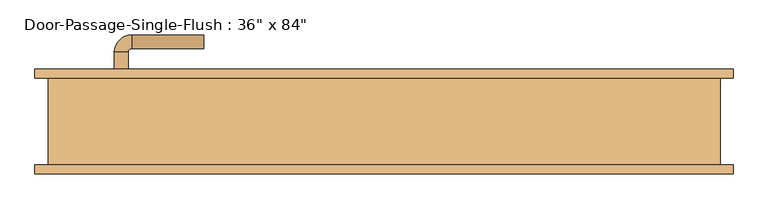
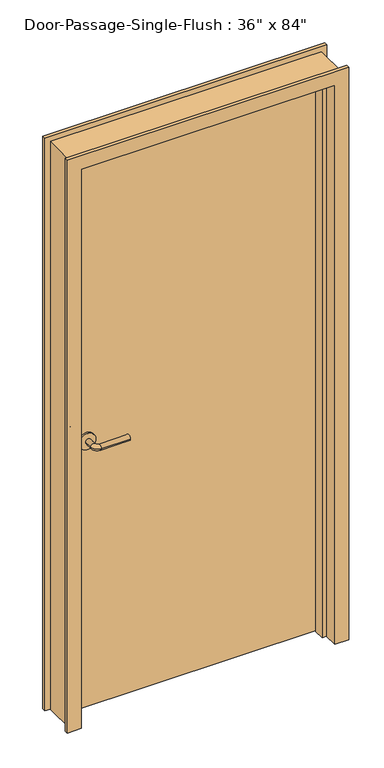
"""IFC4 building model written with IfcOpenShell, lengths in millimetres: door geometry."""

from ifc_helpers import new_model, si_unit, point, frame, frame_2d, origin, origin_with_axes, place, context, project, spatial, polyline, circle_curve, ellipse_curve, trimmed, segment, composite_curve, outline, extrude, faceted_brep, source, transform, mapped, element, save
from ifc_brep_helpers import plane_surface, cylinder_surface, revolved_surface, advanced_brep


def door_12b10c6a(model_context):
    return source(origin(), model_context, "Body", "SolidModel", [
        advanced_brep(
        [(-392.190625, 17.4, 1016.0), (-372.190625, 17.4, 1016.0), (-372.190625, -12.6, 1016.0), (-392.190625, -12.6, 1016.0), (-367.190625, -17.6, 1016.0), (-367.190625, -37.6, 1016.0), (-262.190625, -37.6, 1016.0), (-262.190625, -17.6, 1016.0)],
        [
            (0, 1, circle_curve(frame((-382.190625, 17.4, 1016.0), z_axis=(0.0, 1.0, 0.0), x_axis=(1.0, 0.0, 0.0)), 10.0)),
            (1, 0, circle_curve(frame((-382.190625, 17.4, 1016.0), z_axis=(0.0, 1.0, 0.0), x_axis=(1.0, 0.0, 0.0)), 10.0)),
            (1, 2),
            (2, 3, circle_curve(frame((-382.190625, -12.6, 1016.0), z_axis=(0.0, 1.0, 0.0), x_axis=(1.0, 0.0, 0.0)), 10.0)),
            (3, 0),
            (3, 2, circle_curve(frame((-382.190625, -12.6, 1016.0), z_axis=(0.0, 1.0, 0.0), x_axis=(1.0, 0.0, 0.0)), 10.0)),
            (4, 5, circle_curve(frame((-367.190625, -27.6, 1016.0), z_axis=(-1.0, 0.0, 0.0), x_axis=(0.0, 1.0, 0.0)), 10.0)),
            (5, 3, circle_curve(frame((-367.190625, -12.6, 1016.0), z_axis=(0.0, 0.0, -1.0), x_axis=(-1.0, 0.0, 0.0)), 25.0)),
            (2, 4, circle_curve(frame((-367.190625, -12.6, 1016.0), z_axis=(0.0, 0.0, 1.0), x_axis=(-1.0, 0.0, 0.0)), 5.0)),
            (5, 4, circle_curve(frame((-367.190625, -27.6, 1016.0), z_axis=(-1.0, 0.0, 0.0), x_axis=(0.0, 1.0, 0.0)), 10.0)),
            (6, 7, circle_curve(frame((-262.190625, -27.6, 1016.0), z_axis=(1.0, 0.0, 0.0), x_axis=(0.0, 1.0, 0.0)), 10.0)),
            (7, 6, circle_curve(frame((-262.190625, -27.6, 1016.0), z_axis=(1.0, 0.0, 0.0), x_axis=(0.0, 1.0, 0.0)), 10.0)),
            (4, 7),
            (6, 5),
        ],
        [
            plane_surface(frame((-382.190625, 17.4, 1016.0), z_axis=(0.0, 1.0, 0.0), x_axis=(0.0, 0.0, 1.0))),
            cylinder_surface(frame((-382.190625, 17.4, 1016.0), z_axis=(0.0, 1.0, 0.0), x_axis=(1.0, 0.0, 0.0)), 10.0),
            revolved_surface(trimmed(ellipse_curve(frame((-382.190625, -12.6, 1016.0), z_axis=(0.0, -1.0, 0.0), x_axis=(1.0, 0.0, 0.0)), 10.0, 10.0), [point((-392.190625, -12.6, 1016.0))], [point((-372.190625, -12.6, 1016.0))], True, "CARTESIAN"), (-367.190625, -12.6, 1016.0), (0.0, 0.0, -1.0)),
            revolved_surface(trimmed(ellipse_curve(frame((-382.190625, -12.6, 1016.0), z_axis=(0.0, -1.0, 0.0), x_axis=(1.0, 0.0, 0.0)), 10.0, 10.0), [point((-372.190625, -12.6, 1016.0))], [point((-392.190625, -12.6, 1016.0))], True, "CARTESIAN"), (-367.190625, -12.6, 1016.0), (0.0, 0.0, -1.0)),
            plane_surface(frame((-262.190625, -27.6, 1016.0), z_axis=(1.0, 0.0, 0.0), x_axis=(0.0, 0.0, 1.0))),
            cylinder_surface(frame((-367.190625, -27.6, 1016.0), z_axis=(-1.0, 0.0, 0.0), x_axis=(0.0, 1.0, 0.0)), 10.0),
        ],
        [
            (0, [[1, 2]]),
            (1, [[3, 4, 5, -2]]),
            (1, [[-5, 6, -3, -1]]),
            (2, [[7, 8, -4, 9]]),
            (3, [[10, -9, -6, -8]]),
            (4, [[11, 12]]),
            (5, [[13, -11, 14, -7]]),
            (5, [[-14, -12, -13, -10]]),
        ],
    ),
        extrude(outline(composite_curve([segment(trimmed(circle_curve(frame_2d((1016.0, -384.690625)), 30.0), [point((1016.0, -414.690625))], [point((1016.0, -354.690625))], False, "CARTESIAN"), True, "CONTINUOUS"), segment(trimmed(circle_curve(frame_2d((1016.0, -384.690625)), 30.0), [point((1016.0, -354.690625))], [point((1016.0, -414.690625))], False, "CARTESIAN"), True, "CONTINUOUS")], self_intersect=False)), frame((0.0, 17.4, 0.0), z_axis=(0.0, 1.0, 0.0), x_axis=(0.0, 0.0, 1.0)), (0.0, 0.0, 1.0), 8.0),
        advanced_brep(
        [(-392.190625, 77.85, 1016.0), (-372.190625, 77.85, 1016.0), (-392.190625, 107.85, 1016.0), (-372.190625, 107.85, 1016.0), (-367.190625, 112.85, 1016.0), (-367.190625, 132.85, 1016.0), (-262.190625, 132.85, 1016.0), (-262.190625, 112.85, 1016.0)],
        [
            (0, 1, circle_curve(frame((-382.190625, 77.85, 1016.0), z_axis=(0.0, -1.0, 0.0), x_axis=(1.0, 0.0, 0.0)), 10.0)),
            (1, 0, circle_curve(frame((-382.190625, 77.85, 1016.0), z_axis=(0.0, -1.0, 0.0), x_axis=(1.0, 0.0, 0.0)), 10.0)),
            (0, 2),
            (2, 3, circle_curve(frame((-382.190625, 107.85, 1016.0), z_axis=(0.0, -1.0, 0.0), x_axis=(1.0, 0.0, 0.0)), 10.0)),
            (3, 1),
            (3, 2, circle_curve(frame((-382.190625, 107.85, 1016.0), z_axis=(0.0, -1.0, 0.0), x_axis=(1.0, 0.0, 0.0)), 10.0)),
            (4, 3, circle_curve(frame((-367.190625, 107.85, 1016.0), z_axis=(0.0, 0.0, 1.0), x_axis=(-1.0, 0.0, 0.0)), 5.0)),
            (2, 5, circle_curve(frame((-367.190625, 107.85, 1016.0), z_axis=(0.0, 0.0, -1.0), x_axis=(-1.0, 0.0, 0.0)), 25.0)),
            (5, 4, circle_curve(frame((-367.190625, 122.85, 1016.0), z_axis=(-1.0, 0.0, 0.0), x_axis=(0.0, -1.0, 0.0)), 10.0)),
            (4, 5, circle_curve(frame((-367.190625, 122.85, 1016.0), z_axis=(-1.0, 0.0, 0.0), x_axis=(0.0, -1.0, 0.0)), 10.0)),
            (6, 7, circle_curve(frame((-262.190625, 122.85, 1016.0), z_axis=(1.0, 0.0, 0.0), x_axis=(0.0, -1.0, 0.0)), 10.0)),
            (7, 6, circle_curve(frame((-262.190625, 122.85, 1016.0), z_axis=(1.0, 0.0, 0.0), x_axis=(0.0, -1.0, 0.0)), 10.0)),
            (5, 6),
            (7, 4),
        ],
        [
            plane_surface(frame((-382.190625, 77.85, 1016.0), z_axis=(0.0, -1.0, 0.0), x_axis=(0.0, 0.0, 1.0))),
            cylinder_surface(frame((-382.190625, 77.85, 1016.0), z_axis=(0.0, -1.0, 0.0), x_axis=(1.0, 0.0, 0.0)), 10.0),
            revolved_surface(trimmed(ellipse_curve(frame((-382.190625, 107.85, 1016.0), z_axis=(0.0, -1.0, 0.0), x_axis=(1.0, 0.0, 0.0)), 10.0, 10.0), [point((-392.190625, 107.85, 1016.0))], [point((-372.190625, 107.85, 1016.0))], True, "CARTESIAN"), (-367.190625, 107.85, 1016.0), (0.0, 0.0, -1.0)),
            revolved_surface(trimmed(ellipse_curve(frame((-382.190625, 107.85, 1016.0), z_axis=(0.0, -1.0, 0.0), x_axis=(1.0, 0.0, 0.0)), 10.0, 10.0), [point((-372.190625, 107.85, 1016.0))], [point((-392.190625, 107.85, 1016.0))], True, "CARTESIAN"), (-367.190625, 107.85, 1016.0), (0.0, 0.0, -1.0)),
            plane_surface(frame((-262.190625, 122.85, 1016.0), z_axis=(1.0, 0.0, 0.0), x_axis=(0.0, 0.0, 1.0))),
            cylinder_surface(frame((-367.190625, 122.85, 1016.0), z_axis=(-1.0, 0.0, 0.0), x_axis=(0.0, -1.0, 0.0)), 10.0),
        ],
        [
            (0, [[1, 2]]),
            (1, [[-1, 3, 4, 5]]),
            (1, [[-2, -5, 6, -3]]),
            (2, [[7, -4, 8, 9]]),
            (3, [[-8, -6, -7, 10]]),
            (4, [[11, 12]]),
            (5, [[-9, 13, -12, 14]]),
            (5, [[-10, -14, -11, -13]]),
        ],
    ),
        extrude(outline(composite_curve([segment(trimmed(circle_curve(frame_2d((1016.0, -384.690625)), 30.0), [point((1016.0, -414.690625))], [point((1016.0, -354.690625))], False, "CARTESIAN"), True, "CONTINUOUS"), segment(trimmed(circle_curve(frame_2d((1016.0, -384.690625)), 30.0), [point((1016.0, -354.690625))], [point((1016.0, -414.690625))], False, "CARTESIAN"), True, "CONTINUOUS")], self_intersect=False)), frame((0.0, 69.85, 0.0), z_axis=(0.0, 1.0, 0.0), x_axis=(0.0, 0.0, 1.0)), (0.0, 0.0, 1.0), 8.0),
        faceted_brep([(457.2, 82.55, 0.0), (508.0, 82.55, 0.0), (508.0, 69.85, 0.0), (488.95, 69.85, 0.0), (488.95, -57.15, 0.0), (508.0, -57.15, 0.0), (508.0, -69.85, 0.0), (457.2, -69.85, 0.0), (457.2, -17.4625, 0.0), (441.325, -17.4625, 0.0), (441.325, 20.6375, 0.0), (457.2, 20.6375, 0.0), (457.2, 82.55, 2133.6), (-457.2, 82.55, 2133.6), (-457.2, 82.55, 0.0), (-508.0, 82.55, 0.0), (-508.0, 82.55, 2184.4), (508.0, 82.55, 2184.4), (508.0, 69.85, 2184.4), (-508.0, 69.85, 2184.4), (-508.0, 69.85, 0.0), (-488.95, 69.85, 0.0), (-488.95, 69.85, 2165.35), (488.95, 69.85, 2165.35), (488.95, -57.15, 2165.35), (-488.95, -57.15, 2165.35), (-488.95, -57.15, 0.0), (-508.0, -57.15, 0.0), (-508.0, -57.15, 2184.4), (508.0, -57.15, 2184.4), (508.0, -69.85, 2184.4), (-508.0, -69.85, 2184.4), (-508.0, -69.85, 0.0), (-457.2, -69.85, 0.0), (-457.2, -69.85, 2133.6), (457.2, -69.85, 2133.6), (457.2, -17.4625, 2133.6), (-457.2, -17.4625, 2133.6), (-457.2, -17.4625, 0.0), (-441.325, -17.4625, 0.0), (-441.325, -17.4625, 2117.725), (441.325, -17.4625, 2117.725), (441.325, 20.6375, 2117.725), (-441.325, 20.6375, 2117.725), (-441.325, 20.6375, 0.0), (-457.2, 20.6375, 0.0), (-457.2, 20.6375, 2133.6), (457.2, 20.6375, 2133.6)], [[[0, 1, 2, 3, 4, 5, 6, 7, 8, 9, 10, 11]], [[1, 0, 12, 13, 14, 15, 16, 17]], [[2, 1, 17, 18]], [[3, 2, 18, 19, 20, 21, 22, 23]], [[4, 3, 23, 24]], [[5, 4, 24, 25, 26, 27, 28, 29]], [[6, 5, 29, 30]], [[7, 6, 30, 31, 32, 33, 34, 35]], [[8, 7, 35, 36]], [[9, 8, 36, 37, 38, 39, 40, 41]], [[10, 9, 41, 42]], [[11, 10, 42, 43, 44, 45, 46, 47]], [[0, 11, 47, 12]], [[18, 17, 16, 19]], [[24, 23, 22, 25]], [[30, 29, 28, 31]], [[36, 35, 34, 37]], [[42, 41, 40, 43]], [[12, 47, 46, 13]], [[14, 45, 44, 39, 38, 33, 32, 27, 26, 21, 20, 15]], [[19, 16, 15, 20]], [[25, 22, 21, 26]], [[31, 28, 27, 32]], [[37, 34, 33, 38]], [[43, 40, 39, 44]], [[13, 46, 45, 14]]]),
        extrude(outline(polyline([(457.2, 25.4), (-457.2, 25.4), (-457.2, 69.85), (457.2, 69.85), (457.2, 25.4)])), origin_with_axes(), (0.0, 0.0, 1.0), 2133.6),
    ])


if __name__ == "__main__":
    model = new_model("IFC4")
    model_context = context("Model", 3, world=origin())
    ifc_project = project(units=[si_unit("LENGTHUNIT", "METRE", prefix="MILLI")], contexts=[model_context])
    site = spatial("IfcSite", under=ifc_project)
    building = spatial("IfcBuilding", under=site)
    placement = place(None, origin())
    door_shape = door_12b10c6a(model_context)
    element("IfcDoor", 1, ObjectType="Door-Passage-Single-Flush : 36\" x 84\"", at=placement, inside=building, context=model_context, shape_type="MappedRepresentation", body=[
        mapped(door_shape, transform((0.0, 0.0, 0.0), x_axis=(1.0, 0.0, 0.0), y_axis=(0.0, 1.0, 0.0), z_axis=(0.0, 0.0, 1.0))),
    ])
    save(model, "model.ifc")

# Revit data of these elements
# Type "Door-Passage-Single-Flush : 36\" x 84\""
#   Type Mark = "19"
#   Assembly Code = "B2030200"
#   Analytic Construction = "Wooden"
#   Thickness = 0' - 1 3/4"
#   Thermal Resistance (R) = 2.5876 (h·ft²·°F)/BTU
#   Swing Angle [instance default] = 90.00°
#   Strike Height = 3' - 4"
#   Rough Width [instance default] = 3' - 4"
#   Rough Height [instance default] = 7' - 4"
#   MF Opening Height [instance default] = 0' - 4"
#   MF Opening Width [instance default] = 0' - 4"
#   Inset Calculate [instance default] = 0' - 4"
#   Masonry Inset [instance default] = 0' - 1"
#   Height = 7' - 0"
#   Width = 3' - 0"
#   Heat Transfer Coefficient (U) = 0.3865 BTU/(h·ft²·°F)
#   Masonry Frame Depth = 0' - 5 3/4"
#   Masonry Frame [instance default] = yes
#   Function = 1
#   Dry Wall Frame [instance default] = no
#   Panel Material = Wood - Birch
#   Frame Material = Metal - Paint Finish - Grey
#   Door Handle Material = Aluminum
#   Visual Light Transmittance = 0
#   Solar Heat Gain Coefficient = 0
#   Wall Closure = (empty or 0)
# Element 1 (IfcDoor, "Door-Passage-Single-Flush : 36\" x 84\"")
#   Rough Width = 3' - 2 1/2"
#   Rough Height = 7' - 1 1/4"
#   MF Opening Height = 0' - 1 1/4"
#   MF Opening Width = 0' - 2 1/2"
#   Inset Calculate = 0' - 3"
#   Masonry Frame = no
#   Dry Wall Frame = yes
#   Materials on its faces: "Metal - Paint Finish - Grey", "Aluminum", "Wood - Birch"
# Materials
#   "Wood - Birch": class "Wood", colour RGB 166 116 52, transparency 0, Cost = 0
#   "Metal - Paint Finish - Grey": class "Paint", colour RGB 104 104 104, transparency 0, Cost = 0
#   "Aluminum": class "Metal", colour RGB 247 247 247, transparency 0, Description = "Aluminum 6061", Cost = 0
